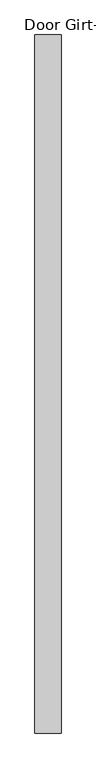
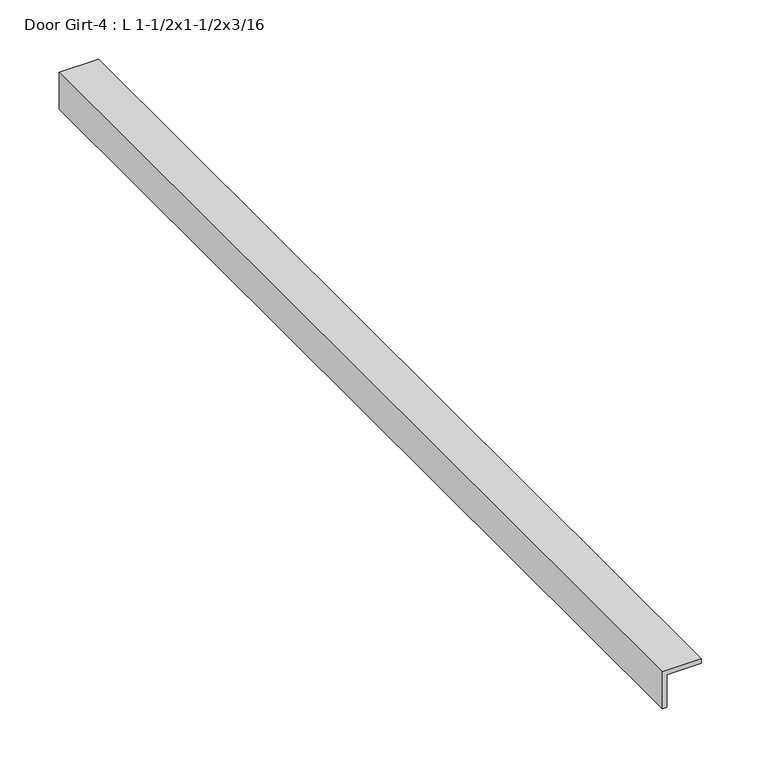
"""IFC4 building model written with IfcOpenShell, lengths in millimetres: proxy geometry, Door Girt-4 : L 1-1/2x1-1/2x3/16."""

from ifc_helpers import new_model, si_unit, frame, origin, place, context, project, spatial, polyline, outline, extrude, source, transform, mapped, element, save


def door_girt_4_l_1_1_2x1_1_2x3_16_602a1831(model_context):
    return source(origin(), model_context, "Body", "SweptSolid", [
        extrude(outline(polyline([(1625.6, 587403.9934739), (1625.6, 587365.8934739), (1587.5, 587365.8934739), (1587.5, 587370.6559739), (1620.8375, 587370.6559739), (1620.8375, 587403.9934739), (1625.6, 587403.9934739)])), frame((0.0, -533937.9163841, 0.0), z_axis=(0.0, 1.0, 0.0), x_axis=(0.0, 0.0, 1.0)), (0.0, 0.0, 1.0), 1016.0),
    ])


if __name__ == "__main__":
    model = new_model("IFC4")
    model_context = context("Model", 3, world=origin())
    ifc_project = project(units=[si_unit("LENGTHUNIT", "METRE", prefix="MILLI")], contexts=[model_context])
    site = spatial("IfcSite", under=ifc_project)
    building = spatial("IfcBuilding", under=site)
    placement = place(None, origin())
    door_girt_4_l_1_1_2x1_1_2x3_16_shape = door_girt_4_l_1_1_2x1_1_2x3_16_602a1831(model_context)
    element("IfcBuildingElementProxy", 1, Name="Door Girt-4 : L 1-1/2x1-1/2x3/16", ObjectType="Door Girt-4 : L 1-1/2x1-1/2x3/16", at=placement, inside=building, context=model_context, shape_type="MappedRepresentation", body=[
        mapped(door_girt_4_l_1_1_2x1_1_2x3_16_shape, transform((0.0, 0.0, 0.0), x_axis=(1.0, 0.0, 0.0), y_axis=(0.0, 1.0, 0.0), z_axis=(0.0, 0.0, 1.0))),
    ])
    save(model, "model.ifc")

# Revit data of these elements
# Element 1 (IfcBuildingElementProxy, "Door Girt-4 : L 1-1/2x1-1/2x3/16")
#   Materials on its faces: "1-1/2\"X1-1/2\" GALV. STL L"
# Materials
#   "1-1/2\"X1-1/2\" GALV. STL L": class "Generic", colour RGB 211 211 207, transparency 0, Cost = 0
